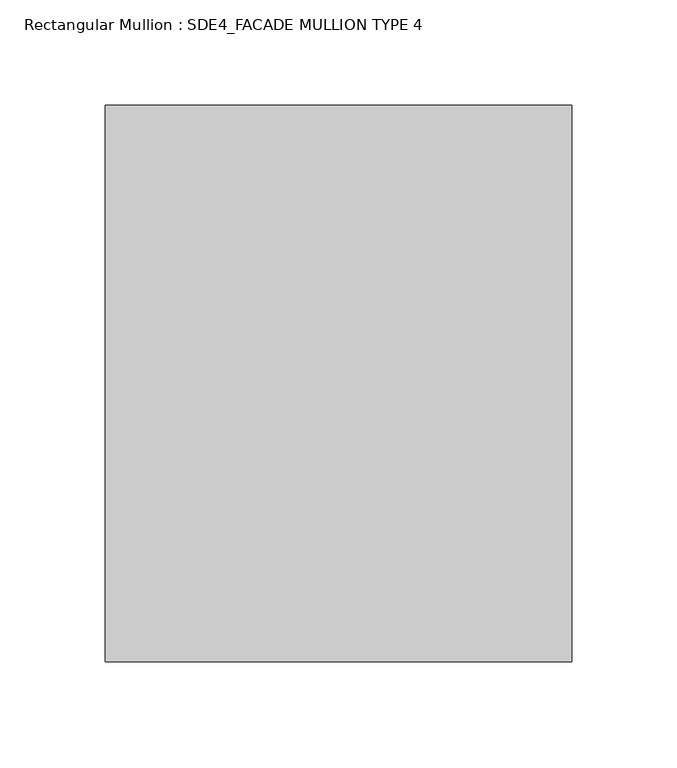
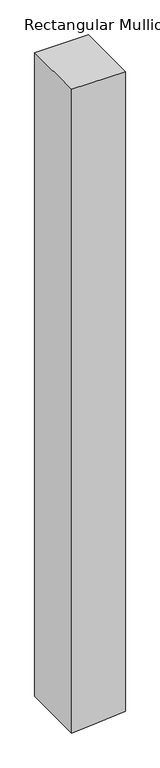
"""IFC4 building model written with IfcOpenShell, lengths in millimetres: member geometry, Rectangular Mullion : SDE4_FACADE MULLION TYPE 4."""

from ifc_helpers import new_model, si_unit, frame, origin, place, context, project, spatial, polyline, outline, extrude, source, transform, mapped, element, save


def rectangular_mullion_sde4_facade_mullion_type_4_5054dcf4(model_context):
    return source(origin(), model_context, "Body", "SweptSolid", [
        extrude(outline(polyline([(0.0, 111.0), (0.0, -111.0), (-2816.8841209, -111.0), (-2808.611681, -3.056508), (-2799.8707594, 111.0), (0.0, 111.0)])), frame((0.0, -132.5, 0.0), z_axis=(0.0, 1.0, 0.0), x_axis=(0.0, 0.0, 1.0)), (0.0, 0.0, 1.0), 265.0),
    ])


if __name__ == "__main__":
    model = new_model("IFC4")
    model_context = context("Model", 3, world=origin())
    ifc_project = project(units=[si_unit("LENGTHUNIT", "METRE", prefix="MILLI")], contexts=[model_context])
    site = spatial("IfcSite", under=ifc_project)
    building = spatial("IfcBuilding", under=site)
    placement = place(None, origin())
    rectangular_mullion_sde4_facade_mullion_type_4_shape = rectangular_mullion_sde4_facade_mullion_type_4_5054dcf4(model_context)
    element("IfcMember", 1, ObjectType="Rectangular Mullion : SDE4_FACADE MULLION TYPE 4", at=placement, inside=building, context=model_context, shape_type="MappedRepresentation", body=[
        mapped(rectangular_mullion_sde4_facade_mullion_type_4_shape, transform((0.0, 0.0, 0.0), x_axis=(1.0, 0.0, 0.0), y_axis=(0.0, 1.0, 0.0), z_axis=(0.0, 0.0, 1.0))),
    ])
    save(model, "model.ifc")

# Revit data of these elements
# Type "Rectangular Mullion : SDE4_FACADE MULLION TYPE 4"
#   built-in parameter 1007322 = 0.869423 (stored number, unit not read)
#   built-in parameter 1007321 = 0.364173 (stored number, unit not read)
#   built-in parameter 1007320 = 0.364173 (stored number, unit not read)
